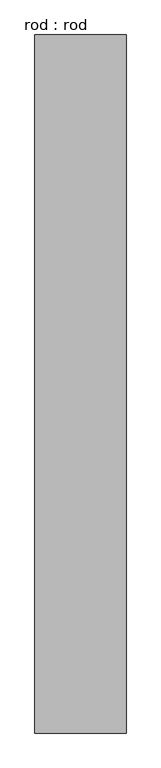
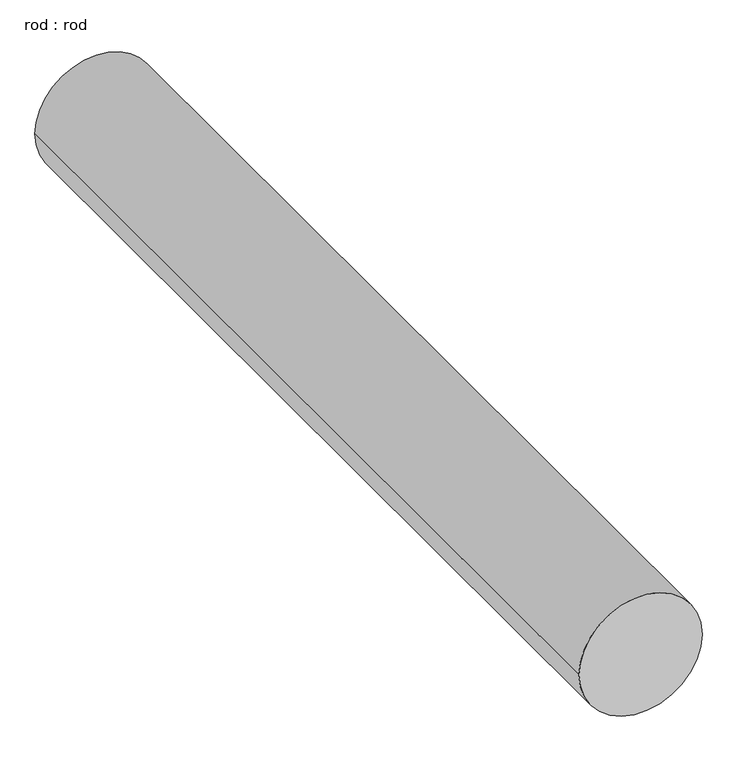
"""IFC4 building model written with IfcOpenShell, lengths in millimetres: proxy geometry, rod : rod."""

from ifc_helpers import new_model, si_unit, point, frame, frame_2d, origin, place, context, project, spatial, circle_curve, trimmed, segment, composite_curve, outline, extrude, source, transform, mapped, element, save


def rod_rod_647cf5a6(model_context):
    return source(origin(), model_context, "Body", "SweptSolid", [
        extrude(outline(composite_curve([segment(trimmed(circle_curve(frame_2d((0.0108462, 0.0)), 200.0), [point((0.0108462, 200.0))], [point((0.0108462, -200.0))], False, "CARTESIAN"), True, "CONTINUOUS"), segment(trimmed(circle_curve(frame_2d((0.0108462, 0.0)), 200.0), [point((0.0108462, -200.0))], [point((0.0108462, 200.0))], False, "CARTESIAN"), True, "CONTINUOUS")], self_intersect=False)), frame((0.0, 2560.5857582, 0.0), z_axis=(0.0, 1.0, 0.0), x_axis=(0.0, 0.0, 1.0)), (0.0, 0.0, 1.0), 3064.2857143),
    ])


if __name__ == "__main__":
    model = new_model("IFC4")
    model_context = context("Model", 3, world=origin())
    ifc_project = project(units=[si_unit("LENGTHUNIT", "METRE", prefix="MILLI")], contexts=[model_context])
    site = spatial("IfcSite", under=ifc_project)
    building = spatial("IfcBuilding", under=site)
    placement = place(None, origin())
    rod_rod_shape = rod_rod_647cf5a6(model_context)
    element("IfcBuildingElementProxy", 1, Name="rod : rod", ObjectType="rod : rod", at=placement, inside=building, context=model_context, shape_type="MappedRepresentation", body=[
        mapped(rod_rod_shape, transform((0.0, 0.0, 0.0), x_axis=(1.0, 0.0, 0.0), y_axis=(0.0, 1.0, 0.0), z_axis=(0.0, 0.0, 1.0))),
    ])
    save(model, "model.ifc")

# Revit data of these elements
# Type "rod : rod"
#   Default Elevation = 0
